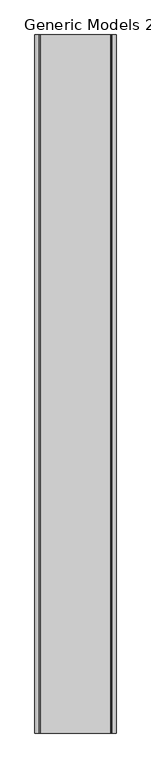
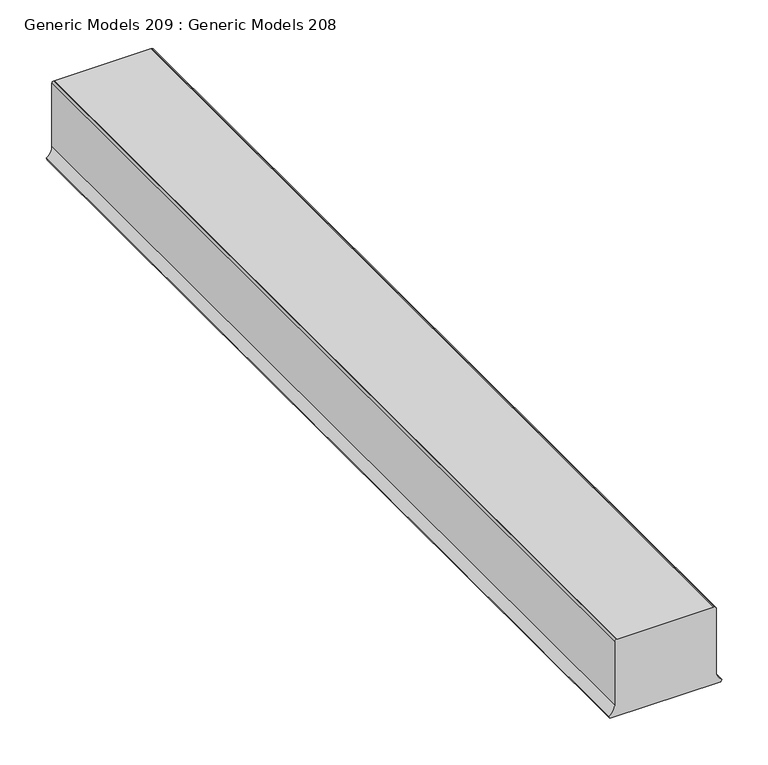
"""IFC4 building model written with IfcOpenShell, lengths in millimetres: proxy geometry, Generic Models 209 : Generic Models 208."""

from ifc_helpers import new_model, si_unit, point, frame, frame_2d, origin, place, context, project, spatial, polyline, circle_curve, trimmed, segment, composite_curve, outline, extrude, source, transform, mapped, element, save


def generic_models_209_generic_models_208_3b29439f(model_context):
    return source(origin(), model_context, "Body", "SweptSolid", [
        extrude(outline(composite_curve([segment(polyline([(101.6, 54929.8579676), (101.6, 54928.7697694)]), True, "CONTINUOUS"), segment(trimmed(circle_curve(frame_2d((99.5131982, 54928.7697694)), 2.0868018), [point((101.6, 54928.7697694))], [point((99.5131982, 54926.6829676))], False, "CARTESIAN"), True, "CONTINUOUS"), segment(polyline([(99.5131982, 54926.6829676), (15.4496307, 54926.6829676)]), True, "CONTINUOUS"), segment(trimmed(circle_curve(frame_2d((15.4496307, 54912.0182708)), 14.6646968), [point((15.4496307, 54926.6829676))], [point((2.7496307, 54919.3506192))], True, "CARTESIAN"), True, "CONTINUOUS"), segment(polyline([(2.7496307, 54919.3506192), (0.0, 54920.9381192), (0.0, 55059.427816), (2.7496307, 55061.015316)]), True, "CONTINUOUS"), segment(trimmed(circle_curve(frame_2d((15.4496307, 55068.3476645)), 14.6646968), [point((2.7496307, 55061.015316))], [point((15.4496307, 55053.6829676))], True, "CARTESIAN"), True, "CONTINUOUS"), segment(polyline([(15.4496307, 55053.6829676), (99.5131982, 55053.6829676)]), True, "CONTINUOUS"), segment(trimmed(circle_curve(frame_2d((99.5131982, 55051.5961658)), 2.0868018), [point((99.5131982, 55053.6829676))], [point((101.6, 55051.5961658))], False, "CARTESIAN"), True, "CONTINUOUS"), segment(polyline([(101.6, 55051.5961658), (101.6, 55050.5079676), (101.6, 54929.8579676)]), True, "CONTINUOUS")], self_intersect=False)), frame((0.0, -228.7033818, 0.0), z_axis=(0.0, 1.0, 0.0), x_axis=(0.0, 0.0, 1.0)), (0.0, 0.0, 1.0), 1219.2),
    ])


if __name__ == "__main__":
    model = new_model("IFC4")
    model_context = context("Model", 3, world=origin())
    ifc_project = project(units=[si_unit("LENGTHUNIT", "METRE", prefix="MILLI")], contexts=[model_context])
    site = spatial("IfcSite", under=ifc_project)
    building = spatial("IfcBuilding", under=site)
    placement = place(None, origin())
    generic_models_209_generic_models_208_shape = generic_models_209_generic_models_208_3b29439f(model_context)
    element("IfcBuildingElementProxy", 1, Name="Generic Models 209 : Generic Models 208", ObjectType="Generic Models 209 : Generic Models 208", at=placement, inside=building, context=model_context, shape_type="MappedRepresentation", body=[
        mapped(generic_models_209_generic_models_208_shape, transform((0.0, 0.0, 0.0), x_axis=(1.0, 0.0, 0.0), y_axis=(0.0, 1.0, 0.0), z_axis=(0.0, 0.0, 1.0))),
    ])
    save(model, "model.ifc")

# Revit data of these elements
# Element 1 (IfcBuildingElementProxy, "Generic Models 209 : Generic Models 208")
#   Materials on its faces: "BASE AS SCHEDULED"
# Materials
#   "BASE AS SCHEDULED": class "Generic", colour RGB 120 120 120, transparency 0, Cost = 0
